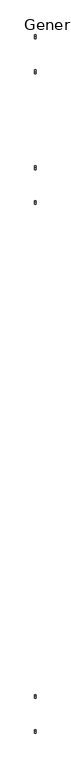
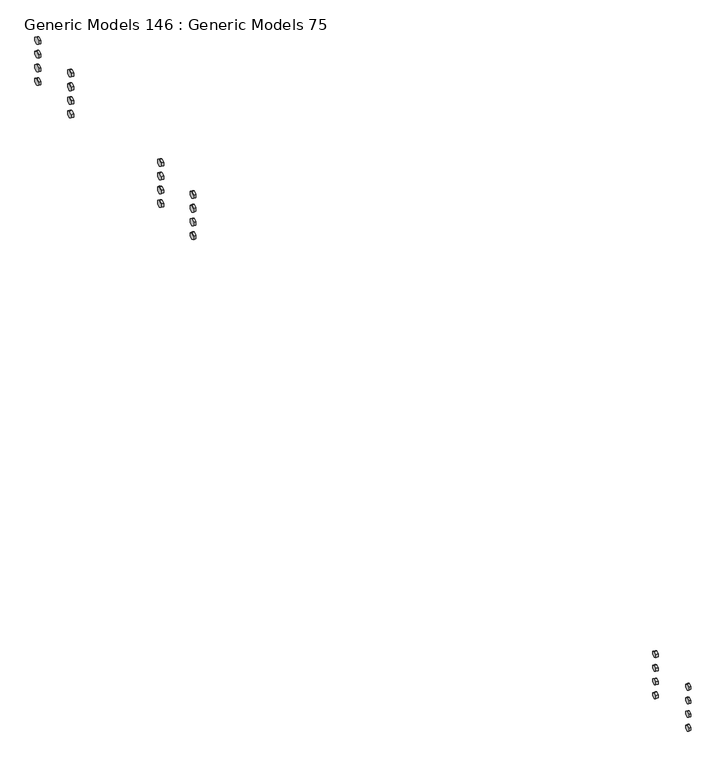
"""IFC4 building model written with IfcOpenShell, lengths in millimetres: proxy geometry, Generic Models 146 : Generic Models 75."""

from ifc_helpers import new_model, si_unit, frame, origin, place, context, project, spatial, polyline, outline, extrude, source, transform, mapped, element, save


def generic_models_146_generic_models_75_f3e5c31a(model_context):
    return source(origin(), model_context, "Body", "SweptSolid", [
        extrude(outline(polyline([(30610.8089892, 268841.8599609), (30625.1156612, 268850.1199219), (30639.4223332, 268841.8599609), (30639.4223332, 268825.3400391), (30625.1156612, 268817.0800781), (30610.8089892, 268825.3400391), (30610.8089892, 268841.8599609)])), frame((32033.3773025, 0.0, 0.0), z_axis=(1.0, 0.0, 0.0), x_axis=(0.0, 1.0, 0.0)), (0.0, 0.0, 1.0), 11.90625),
        extrude(outline(polyline([(30610.8089892, 268918.0599609), (30625.1156612, 268926.3199219), (30639.4223332, 268918.0599609), (30639.4223332, 268901.5400391), (30625.1156612, 268893.2800781), (30610.8089892, 268901.5400391), (30610.8089892, 268918.0599609)])), frame((32033.3773025, 0.0, 0.0), z_axis=(1.0, 0.0, 0.0), x_axis=(0.0, 1.0, 0.0)), (0.0, 0.0, 1.0), 11.90625),
        extrude(outline(polyline([(30610.8089892, 268994.2599609), (30625.1156612, 269002.5199219), (30639.4223332, 268994.2599609), (30639.4223332, 268977.7400391), (30625.1156612, 268969.4800781), (30610.8089892, 268977.7400391), (30610.8089892, 268994.2599609)])), frame((32033.3773025, 0.0, 0.0), z_axis=(1.0, 0.0, 0.0), x_axis=(0.0, 1.0, 0.0)), (0.0, 0.0, 1.0), 11.90625),
        extrude(outline(polyline([(30610.8089892, 269070.4599609), (30625.1156612, 269078.7199219), (30639.4223332, 269070.4599609), (30639.4223332, 269053.9400391), (30625.1156612, 269045.6800781), (30610.8089892, 269053.9400391), (30610.8089892, 269070.4599609)])), frame((32033.3773025, 0.0, 0.0), z_axis=(1.0, 0.0, 0.0), x_axis=(0.0, 1.0, 0.0)), (0.0, 0.0, 1.0), 11.90625),
        extrude(outline(polyline([(30909.2589892, 268841.8599609), (30923.5656612, 268850.1199219), (30937.8723332, 268841.8599609), (30937.8723332, 268825.3400391), (30923.5656612, 268817.0800781), (30909.2589892, 268825.3400391), (30909.2589892, 268841.8599609)])), frame((32033.3773025, 0.0, 0.0), z_axis=(1.0, 0.0, 0.0), x_axis=(0.0, 1.0, 0.0)), (0.0, 0.0, 1.0), 11.90625),
        extrude(outline(polyline([(30909.2589892, 268918.0599609), (30923.5656612, 268926.3199219), (30937.8723332, 268918.0599609), (30937.8723332, 268901.5400391), (30923.5656612, 268893.2800781), (30909.2589892, 268901.5400391), (30909.2589892, 268918.0599609)])), frame((32033.3773025, 0.0, 0.0), z_axis=(1.0, 0.0, 0.0), x_axis=(0.0, 1.0, 0.0)), (0.0, 0.0, 1.0), 11.90625),
        extrude(outline(polyline([(30909.2589892, 268994.2599609), (30923.5656612, 269002.5199219), (30937.8723332, 268994.2599609), (30937.8723332, 268977.7400391), (30923.5656612, 268969.4800781), (30909.2589892, 268977.7400391), (30909.2589892, 268994.2599609)])), frame((32033.3773025, 0.0, 0.0), z_axis=(1.0, 0.0, 0.0), x_axis=(0.0, 1.0, 0.0)), (0.0, 0.0, 1.0), 11.90625),
        extrude(outline(polyline([(35158.6810781, 268995.525), (35158.6810781, 268976.475), (35142.1832942, 268966.95), (35125.6855103, 268976.475), (35125.6855103, 268995.525), (35142.1832942, 269005.05), (35158.6810781, 268995.525)])), frame((32033.3773025, 0.0, 0.0), z_axis=(1.0, 0.0, 0.0), x_axis=(0.0, 1.0, 0.0)), (0.0, 0.0, 1.0), 11.90625),
        extrude(outline(polyline([(35158.6810781, 268919.325), (35158.6810781, 268900.275), (35142.1832942, 268890.75), (35125.6855103, 268900.275), (35125.6855103, 268919.325), (35142.1832942, 268928.85), (35158.6810781, 268919.325)])), frame((32033.3773025, 0.0, 0.0), z_axis=(1.0, 0.0, 0.0), x_axis=(0.0, 1.0, 0.0)), (0.0, 0.0, 1.0), 11.90625),
        extrude(outline(polyline([(36573.1435781, 268843.125), (36573.1435781, 268824.075), (36556.6457942, 268814.55), (36540.1480103, 268824.075), (36540.1480103, 268843.125), (36556.6457942, 268852.65), (36573.1435781, 268843.125)])), frame((32033.3773025, 0.0, 0.0), z_axis=(1.0, 0.0, 0.0), x_axis=(0.0, 1.0, 0.0)), (0.0, 0.0, 1.0), 11.90625),
        extrude(outline(polyline([(36573.1435781, 268919.325), (36573.1435781, 268900.275), (36556.6457942, 268890.75), (36540.1480103, 268900.275), (36540.1480103, 268919.325), (36556.6457942, 268928.85), (36573.1435781, 268919.325)])), frame((32033.3773025, 0.0, 0.0), z_axis=(1.0, 0.0, 0.0), x_axis=(0.0, 1.0, 0.0)), (0.0, 0.0, 1.0), 11.90625),
        extrude(outline(polyline([(36573.1435781, 268995.525), (36573.1435781, 268976.475), (36556.6457942, 268966.95), (36540.1480103, 268976.475), (36540.1480103, 268995.525), (36556.6457942, 269005.05), (36573.1435781, 268995.525)])), frame((32033.3773025, 0.0, 0.0), z_axis=(1.0, 0.0, 0.0), x_axis=(0.0, 1.0, 0.0)), (0.0, 0.0, 1.0), 11.90625),
        extrude(outline(polyline([(36573.1435781, 269071.725), (36573.1435781, 269052.675), (36556.6457942, 269043.15), (36540.1480103, 269052.675), (36540.1480103, 269071.725), (36556.6457942, 269081.25), (36573.1435781, 269071.725)])), frame((32033.3773025, 0.0, 0.0), z_axis=(1.0, 0.0, 0.0), x_axis=(0.0, 1.0, 0.0)), (0.0, 0.0, 1.0), 11.90625),
        extrude(outline(polyline([(36274.6935781, 268843.125), (36274.6935781, 268824.075), (36258.1957942, 268814.55), (36241.6980103, 268824.075), (36241.6980103, 268843.125), (36258.1957942, 268852.65), (36274.6935781, 268843.125)])), frame((32033.3773025, 0.0, 0.0), z_axis=(1.0, 0.0, 0.0), x_axis=(0.0, 1.0, 0.0)), (0.0, 0.0, 1.0), 11.90625),
        extrude(outline(polyline([(36274.6935781, 268919.325), (36274.6935781, 268900.275), (36258.1957942, 268890.75), (36241.6980103, 268900.275), (36241.6980103, 268919.325), (36258.1957942, 268928.85), (36274.6935781, 268919.325)])), frame((32033.3773025, 0.0, 0.0), z_axis=(1.0, 0.0, 0.0), x_axis=(0.0, 1.0, 0.0)), (0.0, 0.0, 1.0), 11.90625),
        extrude(outline(polyline([(36274.6935781, 268995.525), (36274.6935781, 268976.475), (36258.1957942, 268966.95), (36241.6980103, 268976.475), (36241.6980103, 268995.525), (36258.1957942, 269005.05), (36274.6935781, 268995.525)])), frame((32033.3773025, 0.0, 0.0), z_axis=(1.0, 0.0, 0.0), x_axis=(0.0, 1.0, 0.0)), (0.0, 0.0, 1.0), 11.90625),
        extrude(outline(polyline([(36274.6935781, 269071.725), (36274.6935781, 269052.675), (36258.1957942, 269043.15), (36241.6980103, 269052.675), (36241.6980103, 269071.725), (36258.1957942, 269081.25), (36274.6935781, 269071.725)])), frame((32033.3773025, 0.0, 0.0), z_axis=(1.0, 0.0, 0.0), x_axis=(0.0, 1.0, 0.0)), (0.0, 0.0, 1.0), 11.90625),
        extrude(outline(polyline([(35453.9560781, 268843.125), (35453.9560781, 268824.075), (35437.4582942, 268814.55), (35420.9605103, 268824.075), (35420.9605103, 268843.125), (35437.4582942, 268852.65), (35453.9560781, 268843.125)])), frame((32033.3773025, 0.0, 0.0), z_axis=(1.0, 0.0, 0.0), x_axis=(0.0, 1.0, 0.0)), (0.0, 0.0, 1.0), 11.90625),
        extrude(outline(polyline([(35453.9560781, 268919.325), (35453.9560781, 268900.275), (35437.4582942, 268890.75), (35420.9605103, 268900.275), (35420.9605103, 268919.325), (35437.4582942, 268928.85), (35453.9560781, 268919.325)])), frame((32033.3773025, 0.0, 0.0), z_axis=(1.0, 0.0, 0.0), x_axis=(0.0, 1.0, 0.0)), (0.0, 0.0, 1.0), 11.90625),
        extrude(outline(polyline([(35453.9560781, 268995.525), (35453.9560781, 268976.475), (35437.4582942, 268966.95), (35420.9605103, 268976.475), (35420.9605103, 268995.525), (35437.4582942, 269005.05), (35453.9560781, 268995.525)])), frame((32033.3773025, 0.0, 0.0), z_axis=(1.0, 0.0, 0.0), x_axis=(0.0, 1.0, 0.0)), (0.0, 0.0, 1.0), 11.90625),
        extrude(outline(polyline([(35453.9560781, 269071.725), (35453.9560781, 269052.675), (35437.4582942, 269043.15), (35420.9605103, 269052.675), (35420.9605103, 269071.725), (35437.4582942, 269081.25), (35453.9560781, 269071.725)])), frame((32033.3773025, 0.0, 0.0), z_axis=(1.0, 0.0, 0.0), x_axis=(0.0, 1.0, 0.0)), (0.0, 0.0, 1.0), 11.90625),
        extrude(outline(polyline([(35158.6810781, 268843.125), (35158.6810781, 268824.075), (35142.1832942, 268814.55), (35125.6855103, 268824.075), (35125.6855103, 268843.125), (35142.1832942, 268852.65), (35158.6810781, 268843.125)])), frame((32033.3773025, 0.0, 0.0), z_axis=(1.0, 0.0, 0.0), x_axis=(0.0, 1.0, 0.0)), (0.0, 0.0, 1.0), 11.90625),
        extrude(outline(polyline([(35158.6810781, 269071.725), (35158.6810781, 269052.675), (35142.1832942, 269043.15), (35125.6855103, 269052.675), (35125.6855103, 269071.725), (35142.1832942, 269081.25), (35158.6810781, 269071.725)])), frame((32033.3773025, 0.0, 0.0), z_axis=(1.0, 0.0, 0.0), x_axis=(0.0, 1.0, 0.0)), (0.0, 0.0, 1.0), 11.90625),
        extrude(outline(polyline([(30909.2589892, 269070.4599609), (30923.5656612, 269078.7199219), (30937.8723332, 269070.4599609), (30937.8723332, 269053.9400391), (30923.5656612, 269045.6800781), (30909.2589892, 269053.9400391), (30909.2589892, 269070.4599609)])), frame((32033.3773025, 0.0, 0.0), z_axis=(1.0, 0.0, 0.0), x_axis=(0.0, 1.0, 0.0)), (0.0, 0.0, 1.0), 11.90625),
    ])


if __name__ == "__main__":
    model = new_model("IFC4")
    model_context = context("Model", 3, world=origin())
    ifc_project = project(units=[si_unit("LENGTHUNIT", "METRE", prefix="MILLI")], contexts=[model_context])
    site = spatial("IfcSite", under=ifc_project)
    building = spatial("IfcBuilding", under=site)
    placement = place(None, origin())
    generic_models_146_generic_models_75_shape = generic_models_146_generic_models_75_f3e5c31a(model_context)
    element("IfcBuildingElementProxy", 1, Name="Generic Models 146 : Generic Models 75", ObjectType="Generic Models 146 : Generic Models 75", at=placement, inside=building, context=model_context, shape_type="MappedRepresentation", body=[
        mapped(generic_models_146_generic_models_75_shape, transform((0.0, 0.0, 0.0), x_axis=(1.0, 0.0, 0.0), y_axis=(0.0, 1.0, 0.0), z_axis=(0.0, 0.0, 1.0))),
    ])
    save(model, "model.ifc")

# Revit data of these elements
# Element 1 (IfcBuildingElementProxy, "Generic Models 146 : Generic Models 75")
#   Materials on its faces: "3/4\" DIA LAG BOLTS"
# Materials
#   "3/4\" DIA LAG BOLTS": class "Generic", colour RGB 255 255 0, transparency 0, Cost = 0
